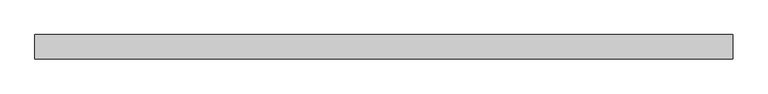
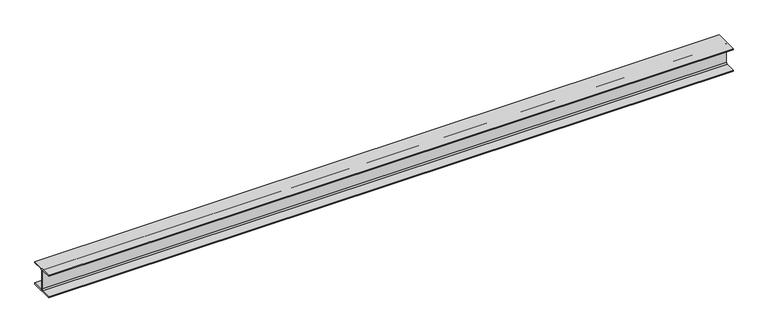
"""IFC4 building model written with IfcOpenShell, lengths in millimetres: beam geometry, 0912_Steel Framing_H-KSD3502 : H_SB_ASB_H-300x300x10x15."""

from ifc_helpers import new_model, si_unit, point, frame, frame_2d, origin, place, context, project, spatial, polyline, circle_curve, trimmed, segment, composite_curve, outline, extrude, source, transform, mapped, element, save


def beam_587d2a9e(model_context):
    return source(origin(), model_context, "Body", "SweptSolid", [
        extrude(outline(composite_curve([segment(polyline([(150.0, -135.0), (150.0, -150.0), (-150.0, -150.0), (-150.0, -135.0), (-23.0, -135.0)]), True, "CONTINUOUS"), segment(trimmed(circle_curve(frame_2d((-23.0, -117.0)), 18.0), [point((-23.0, -135.0))], [point((-5.0, -117.0))], True, "CARTESIAN"), True, "CONTINUOUS"), segment(polyline([(-5.0, -117.0), (-5.0, 117.0)]), True, "CONTINUOUS"), segment(trimmed(circle_curve(frame_2d((-23.0, 117.0)), 18.0), [point((-5.0, 117.0))], [point((-23.0, 135.0))], True, "CARTESIAN"), True, "CONTINUOUS"), segment(polyline([(-23.0, 135.0), (-150.0, 135.0), (-150.0, 150.0), (150.0, 150.0), (150.0, 135.0), (23.0, 135.0)]), True, "CONTINUOUS"), segment(trimmed(circle_curve(frame_2d((23.0, 117.0)), 18.0), [point((23.0, 135.0))], [point((5.0, 117.0))], True, "CARTESIAN"), True, "CONTINUOUS"), segment(polyline([(5.0, 117.0), (5.0, -117.0)]), True, "CONTINUOUS"), segment(trimmed(circle_curve(frame_2d((23.0, -117.0)), 18.0), [point((5.0, -117.0))], [point((23.0, -135.0))], True, "CARTESIAN"), True, "CONTINUOUS"), segment(polyline([(23.0, -135.0), (150.0, -135.0)]), True, "CONTINUOUS")], self_intersect=False)), frame((-4328.9958952, 0.0, 0.0), z_axis=(1.0, 0.0, 0.0), x_axis=(0.0, 1.0, 0.0)), (0.0, 0.0, 1.0), 8601.9210734),
    ])


if __name__ == "__main__":
    model = new_model("IFC4")
    model_context = context("Model", 3, world=origin())
    ifc_project = project(units=[si_unit("LENGTHUNIT", "METRE", prefix="MILLI")], contexts=[model_context])
    site = spatial("IfcSite", under=ifc_project)
    building = spatial("IfcBuilding", under=site)
    placement = place(None, origin())
    beam_shape = beam_587d2a9e(model_context)
    element("IfcBeam", 1, ObjectType="0912_Steel Framing_H-KSD3502 : H_SB_ASB_H-300x300x10x15", at=placement, inside=building, context=model_context, shape_type="MappedRepresentation", body=[
        mapped(beam_shape, transform((0.0, 0.0, 0.0), x_axis=(1.0, 0.0, 0.0), y_axis=(0.0, 1.0, 0.0), z_axis=(0.0, 0.0, 1.0))),
    ])
    save(model, "model.ifc")

# Revit data of these elements
# Type "0912_Steel Framing_H-KSD3502 : H_SB_ASB_H-300x300x10x15"
#   H_WM Code_1 = "S01AA001-00001 | Main Steel Structure Fabrication Work | Shelter/Building | Heavy Steel - Standard (Weight≥90KG/M) | Material: (   )"
#   H_WM Code_2 = "S03AA027-00001 | Main Steel Structure Erection Work | Shelter/Building | Heavy Steel (Weight≥90KG/M) | Material: (   )"
#   H_WM Code_3 = "S01AA010-00001 | Main Steel Structure Fabrication Work | Shelter/Building | Steel Painting/Coating | for Non-Fireproofed Steel Surface, Surface Preparation, Primer, Second & Final Coat | Material: (   )"
#   H_Q'ty Cal Type Tag = "SB-Q2"
#   Width = 30.0 cm
#   Web Thickness = 1.0 cm
#   Web Fillet = 1.8 cm
#   Warping Constant = 1370000.0 cm⁶
#   W = 0
#   Torsional Moment of Inertia = 77.00 cm⁴
#   Section Area = 119.8 cm²
#   Plastic Modulus weak axis = 684.0 cm³
#   Plastic Modulus strong axis = 1500.0 cm³
#   Perimeter = 1.75 m²/m
#   Nominal Weight = 94.00 kgf/m
#   Moment of Inertia weak axis = 6750.00 cm⁴
#   Moment of Inertia strong axis = 20400.00 cm⁴
#   Height = 30.0 cm
#   Flange Thickness = 1.5 cm
#   Elastic Modulus weak axis = 450.0 cm³
#   Elastic Modulus strong axis = 1360.0 cm³
#   Centroid Vertical = 15.0 cm
#   Centroid Horizontal = 15.0 cm
#   Ix = 204000000
#   Length [instance default] = 1.5240 m
#   Zx = 1500000
#   b = 0.3000 m
#   h = 0.3000 m
#   r = 0.0180 m
#   s = 0.0100 m
#   t = 0.0150 m
#   A = 0.01198 m²
#   Structural Material [instance default] = Steel, 45-345
#   Assembly Code = ""
# Element 1 (IfcBeam, "0912_Steel Framing_H-KSD3502 : H_SB_ASB_H-300x300x10x15")
#   Structural Material = none
# Materials
#   "Steel, 45-345": class "Metal", colour RGB 189 187 185, transparency 0, Description = "Steel 345 MPa", Cost = 0
